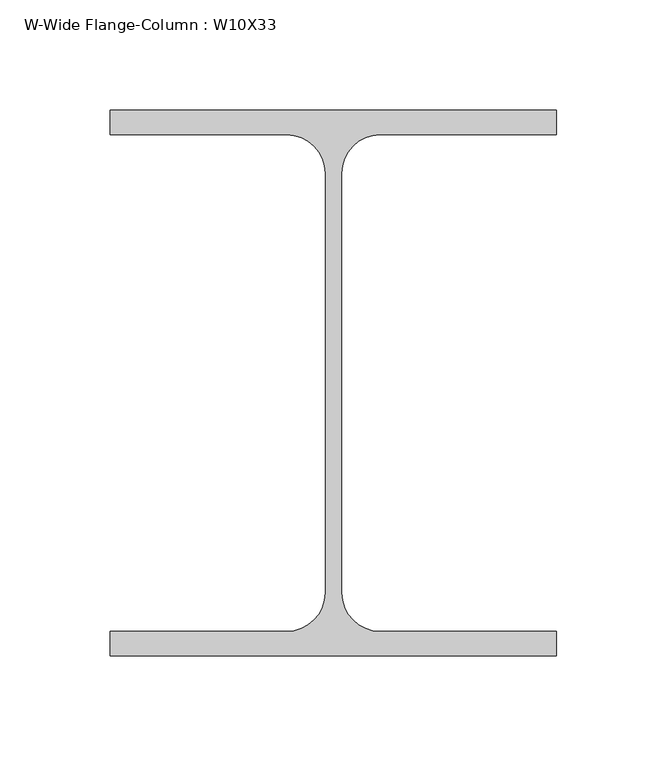
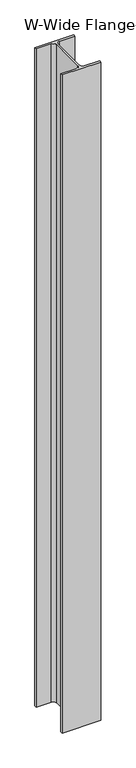
"""IFC4 building model written with IfcOpenShell, lengths in millimetres: column geometry, W-Wide Flange-Column : W10X33."""

from ifc_helpers import new_model, si_unit, point, frame, frame_2d, origin, place, context, project, spatial, polyline, circle_curve, trimmed, segment, composite_curve, outline, extrude, source, transform, mapped, element, save


def w_wide_flange_column_w10x33_4909dbaa(model_context):
    return source(origin(), model_context, "Body", "SweptSolid", [
        extrude(outline(composite_curve([segment(polyline([(101.092, 123.571), (101.092, 112.522), (21.209, 112.522)]), True, "CONTINUOUS"), segment(trimmed(circle_curve(frame_2d((21.209, 94.996)), 17.526), [point((21.209, 112.522))], [point((3.683, 94.996))], True, "CARTESIAN"), True, "CONTINUOUS"), segment(polyline([(3.683, 94.996), (3.683, -94.996)]), True, "CONTINUOUS"), segment(trimmed(circle_curve(frame_2d((21.209, -94.996)), 17.526), [point((3.683, -94.996))], [point((21.209, -112.522))], True, "CARTESIAN"), True, "CONTINUOUS"), segment(polyline([(21.209, -112.522), (101.092, -112.522), (101.092, -123.571), (-101.092, -123.571), (-101.092, -112.522), (-21.209, -112.522)]), True, "CONTINUOUS"), segment(trimmed(circle_curve(frame_2d((-21.209, -94.996)), 17.526), [point((-21.209, -112.522))], [point((-3.683, -94.996))], True, "CARTESIAN"), True, "CONTINUOUS"), segment(polyline([(-3.683, -94.996), (-3.683, 94.996)]), True, "CONTINUOUS"), segment(trimmed(circle_curve(frame_2d((-21.209, 94.996)), 17.526), [point((-3.683, 94.996))], [point((-21.209, 112.522))], True, "CARTESIAN"), True, "CONTINUOUS"), segment(polyline([(-21.209, 112.522), (-101.092, 112.522), (-101.092, 123.571), (101.092, 123.571)]), True, "CONTINUOUS")], self_intersect=False)), frame((0.0, 0.0, 12566.65), z_axis=(0.0, 0.0, 1.0), x_axis=(1.0, 0.0, 0.0)), (0.0, 0.0, 1.0), 3638.55),
    ])


if __name__ == "__main__":
    model = new_model("IFC4")
    model_context = context("Model", 3, world=origin())
    ifc_project = project(units=[si_unit("LENGTHUNIT", "METRE", prefix="MILLI")], contexts=[model_context])
    site = spatial("IfcSite", under=ifc_project)
    building = spatial("IfcBuilding", under=site)
    placement = place(None, origin())
    w_wide_flange_column_w10x33_shape = w_wide_flange_column_w10x33_4909dbaa(model_context)
    element("IfcColumn", 1, ObjectType="W-Wide Flange-Column : W10X33", at=placement, inside=building, context=model_context, shape_type="MappedRepresentation", body=[
        mapped(w_wide_flange_column_w10x33_shape, transform((0.0, 0.0, 0.0), x_axis=(1.0, 0.0, 0.0), y_axis=(0.0, 1.0, 0.0), z_axis=(0.0, 0.0, 1.0))),
    ])
    save(model, "model.ifc")

# Revit data of these elements
# Type "W-Wide Flange-Column : W10X33"
#   Assembly Code = "B10"
#   W = 33
#   bf = 0' - 7.96"
#   d = 0' - 9.73"
#   k = 0' - 1 1/8"
#   kr = 0' - 0.69"
#   tf = 0' - 0.435"
#   tw = 0' - 0.29"
#   A = 0.0674306 SF
#   Structural Material [instance default] = Steel ASTM A992
# Element 1 (IfcColumn, "W-Wide Flange-Column : W10X33")
#   Materials on its faces: "Steel ASTM A992"
# Materials
#   "Steel ASTM A992": class "Metal", colour RGB 199 199 199, transparency 0, Description = "Structural steel 50ksi", Cost = 0
